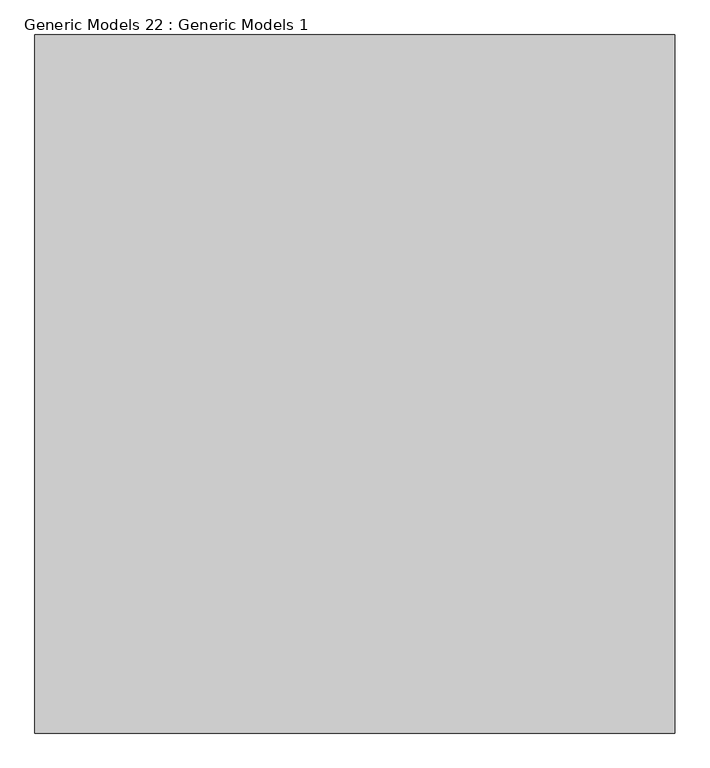
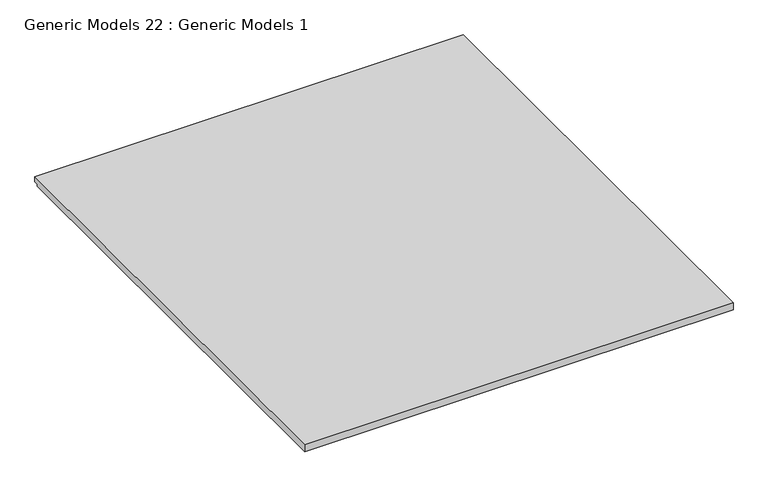
"""IFC4 building model written with IfcOpenShell, lengths in millimetres: proxy geometry, Generic Models 22 : Generic Models 1."""

from ifc_helpers import new_model, si_unit, frame, origin, place, context, project, spatial, polyline, outline, extrude, source, transform, mapped, element, save


def generic_models_22_generic_models_1_6d5e8706(model_context):
    return source(origin(), model_context, "Body", "SweptSolid", [
        extrude(outline(polyline([(39401.9558622, 2631.6803942), (39401.9558622, 2617.3928942), (39390.9627308, 2617.3928942), (39390.9627308, 2612.6303942), (38182.7558622, 2612.6303942), (38182.7558622, 2631.6803942), (39401.9558622, 2631.6803942)])), frame((51480.3077305, 0.0, 0.0), z_axis=(1.0, 0.0, 0.0), x_axis=(0.0, 1.0, 0.0)), (0.0, 0.0, 1.0), 1117.6),
    ])


if __name__ == "__main__":
    model = new_model("IFC4")
    model_context = context("Model", 3, world=origin())
    ifc_project = project(units=[si_unit("LENGTHUNIT", "METRE", prefix="MILLI")], contexts=[model_context])
    site = spatial("IfcSite", under=ifc_project)
    building = spatial("IfcBuilding", under=site)
    placement = place(None, origin())
    generic_models_22_generic_models_1_shape = generic_models_22_generic_models_1_6d5e8706(model_context)
    element("IfcBuildingElementProxy", 1, Name="Generic Models 22 : Generic Models 1", ObjectType="Generic Models 22 : Generic Models 1", at=placement, inside=building, context=model_context, shape_type="MappedRepresentation", body=[
        mapped(generic_models_22_generic_models_1_shape, transform((0.0, 0.0, 0.0), x_axis=(1.0, 0.0, 0.0), y_axis=(0.0, 1.0, 0.0), z_axis=(0.0, 0.0, 1.0))),
    ])
    save(model, "model.ifc")

# Revit data of these elements
# Element 1 (IfcBuildingElementProxy, "Generic Models 22 : Generic Models 1")
#   Materials on its faces: "EXISTING ACOUSTICAL TILE"
# Materials
#   "EXISTING ACOUSTICAL TILE": class "Generic", colour RGB 120 120 120, transparency 0, Cost = 0
